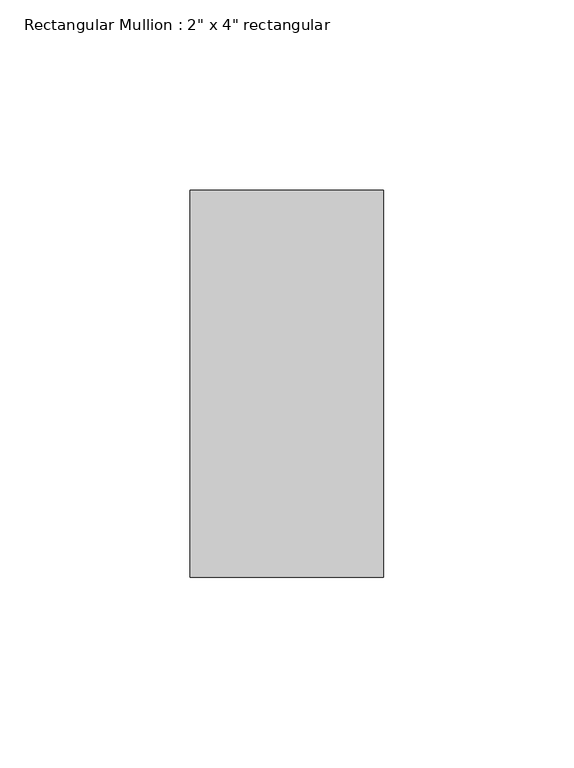
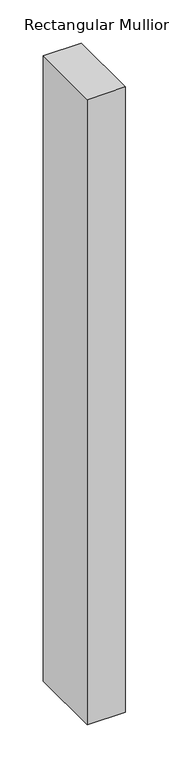
"""IFC4 building model written with IfcOpenShell, lengths in millimetres: member geometry."""

from ifc_helpers import new_model, si_unit, frame, origin, place, context, project, spatial, polyline, outline, extrude, source, transform, mapped, element, save


def member_fdc0e404(model_context):
    return source(origin(), model_context, "Body", "SweptSolid", [
        extrude(outline(polyline([(0.0, 50.8), (0.0, -50.8), (-50.8, -50.8), (-50.8, 50.8), (0.0, 50.8)])), frame((0.0, 0.0, -881.7428574), z_axis=(0.0, 0.0, 1.0), x_axis=(1.0, 0.0, 0.0)), (0.0, 0.0, 1.0), 881.7428574),
    ])


if __name__ == "__main__":
    model = new_model("IFC4")
    model_context = context("Model", 3, world=origin())
    ifc_project = project(units=[si_unit("LENGTHUNIT", "METRE", prefix="MILLI")], contexts=[model_context])
    site = spatial("IfcSite", under=ifc_project)
    building = spatial("IfcBuilding", under=site)
    placement = place(None, origin())
    member_shape = member_fdc0e404(model_context)
    element("IfcMember", 1, ObjectType="Rectangular Mullion : 2\" x 4\" rectangular", at=placement, inside=building, context=model_context, shape_type="MappedRepresentation", body=[
        mapped(member_shape, transform((0.0, 0.0, 0.0), x_axis=(1.0, 0.0, 0.0), y_axis=(0.0, 1.0, 0.0), z_axis=(0.0, 0.0, 1.0))),
    ])
    save(model, "model.ifc")

# Revit data of these elements
# Type "Rectangular Mullion : 2\" x 4\" rectangular"
#   built-in parameter 1007304 = 0.333333 (stored number, unit not read)
#   built-in parameter 1007301 = 0.0833333 (stored number, unit not read)
#   built-in parameter 1007300 = 0.0833333 (stored number, unit not read)
